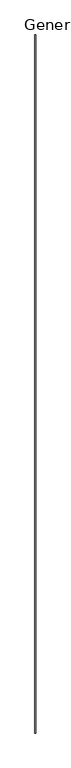
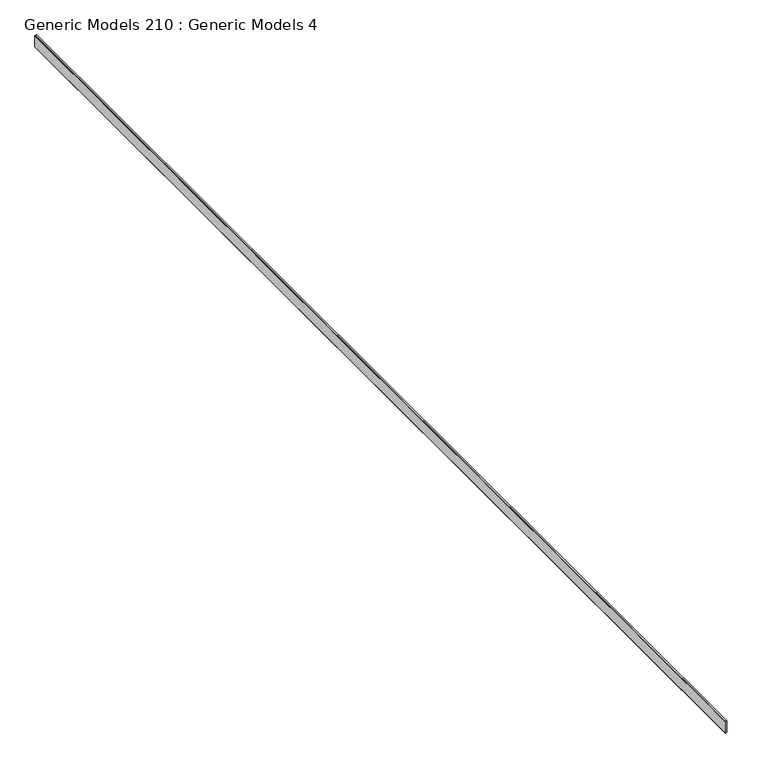
"""IFC4 building model written with IfcOpenShell, lengths in millimetres: proxy geometry, Generic Models 210 : Generic Models 4."""

from ifc_helpers import new_model, si_unit, frame, origin, place, context, project, spatial, polyline, outline, extrude, source, transform, mapped, element, save


def generic_models_210_generic_models_4_0c666629(model_context):
    return source(origin(), model_context, "Body", "SweptSolid", [
        extrude(outline(polyline([(126194.3578287, -6629.7612592), (126322.201, -6629.7612592), (126322.201, -6646.8112339), (126318.7212, -6646.8112339), (126318.7212, -6648.0812339), (126197.8376287, -6648.0812339), (126197.8376287, -6647.222393), (126216.8822074, -6647.222393), (126216.8822074, -6645.952393), (126196.5676287, -6645.952393), (126196.5676287, -6646.8112339), (126194.3578287, -6646.8112339), (126194.3578287, -6629.7612592)])), frame((0.0, -464.1230338, 0.0), z_axis=(0.0, 1.0, 0.0), x_axis=(0.0, 0.0, 1.0)), (0.0, 0.0, 1.0), 12242.8),
    ])


if __name__ == "__main__":
    model = new_model("IFC4")
    model_context = context("Model", 3, world=origin())
    ifc_project = project(units=[si_unit("LENGTHUNIT", "METRE", prefix="MILLI")], contexts=[model_context])
    site = spatial("IfcSite", under=ifc_project)
    building = spatial("IfcBuilding", under=site)
    placement = place(None, origin())
    generic_models_210_generic_models_4_shape = generic_models_210_generic_models_4_0c666629(model_context)
    element("IfcBuildingElementProxy", 1, Name="Generic Models 210 : Generic Models 4", ObjectType="Generic Models 210 : Generic Models 4", at=placement, inside=building, context=model_context, shape_type="MappedRepresentation", body=[
        mapped(generic_models_210_generic_models_4_shape, transform((0.0, 0.0, 0.0), x_axis=(1.0, 0.0, 0.0), y_axis=(0.0, 1.0, 0.0), z_axis=(0.0, 0.0, 1.0))),
    ])
    save(model, "model.ifc")

# Revit data of these elements
# Element 1 (IfcBuildingElementProxy, "Generic Models 210 : Generic Models 4")
#   Materials on its faces: "_7/8\" SMOOTH TROWEL EXTERIOR STUCCO (COLOR PER OWNER)"
# Materials
#   "_7/8\" SMOOTH TROWEL EXTERIOR STUCCO (COLOR PER OWNER)": class "Generic", colour RGB 233 233 233, transparency 0, Cost = 0
